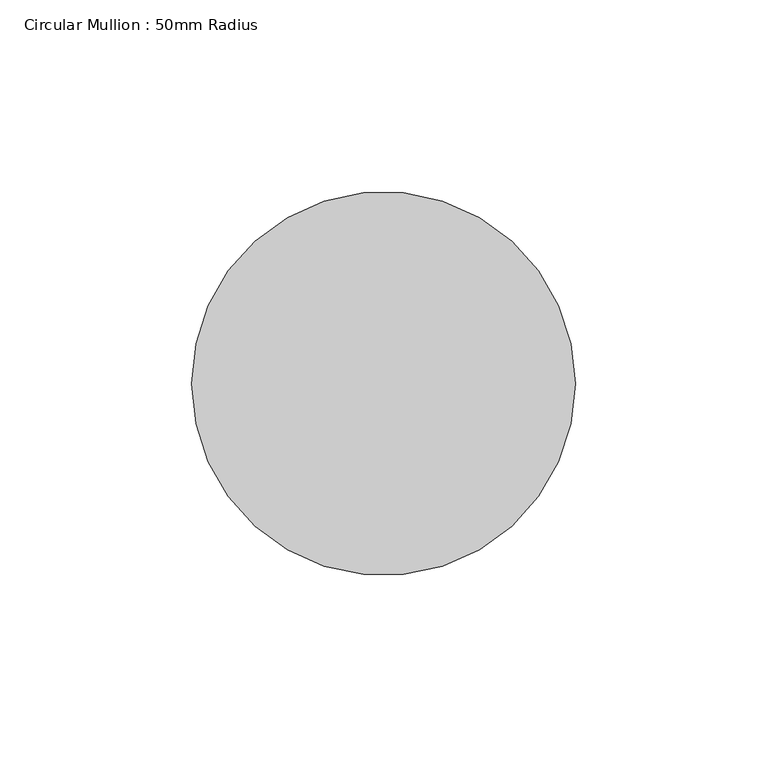
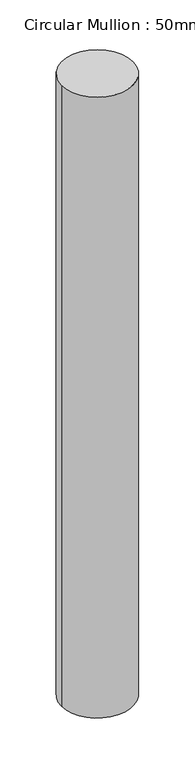
"""IFC4 building model written with IfcOpenShell, lengths in millimetres: member geometry, Circular Mullion : 50mm Radius."""

from ifc_helpers import new_model, si_unit, point, frame, origin, origin_2d, place, context, project, spatial, circle_curve, trimmed, segment, composite_curve, outline, extrude, source, transform, mapped, element, save


def circular_mullion_50mm_radius_81b29c79(model_context):
    return source(origin(), model_context, "Body", "SweptSolid", [
        extrude(outline(composite_curve([segment(trimmed(circle_curve(origin_2d(), 50.0), [point((50.0, 0.0))], [point((-50.0, 0.0))], False, "CARTESIAN"), True, "CONTINUOUS"), segment(trimmed(circle_curve(origin_2d(), 50.0), [point((-50.0, 0.0))], [point((50.0, 0.0))], False, "CARTESIAN"), True, "CONTINUOUS")], self_intersect=False)), frame((0.0, 0.0, -919.7022726), z_axis=(0.0, 0.0, 1.0), x_axis=(1.0, 0.0, 0.0)), (0.0, 0.0, 1.0), 919.7022726),
    ])


if __name__ == "__main__":
    model = new_model("IFC4")
    model_context = context("Model", 3, world=origin())
    ifc_project = project(units=[si_unit("LENGTHUNIT", "METRE", prefix="MILLI")], contexts=[model_context])
    site = spatial("IfcSite", under=ifc_project)
    building = spatial("IfcBuilding", under=site)
    placement = place(None, origin())
    circular_mullion_50mm_radius_shape = circular_mullion_50mm_radius_81b29c79(model_context)
    element("IfcMember", 1, ObjectType="Circular Mullion : 50mm Radius", at=placement, inside=building, context=model_context, shape_type="MappedRepresentation", body=[
        mapped(circular_mullion_50mm_radius_shape, transform((0.0, 0.0, 0.0), x_axis=(1.0, 0.0, 0.0), y_axis=(0.0, 1.0, 0.0), z_axis=(0.0, 0.0, 1.0))),
    ])
    save(model, "model.ifc")

# Revit data of these elements
# Type "Circular Mullion : 50mm Radius"
#   built-in parameter 1007350 = 0.164042 (stored number, unit not read)
# Element 1 (IfcMember, "Circular Mullion : 50mm Radius")
#   Materials on its faces: "Aluminium"
# Materials
#   "Aluminium": class "Metal", colour RGB 247 247 247, transparency 0, Description = "Aluminium 6061", Cost = 0
